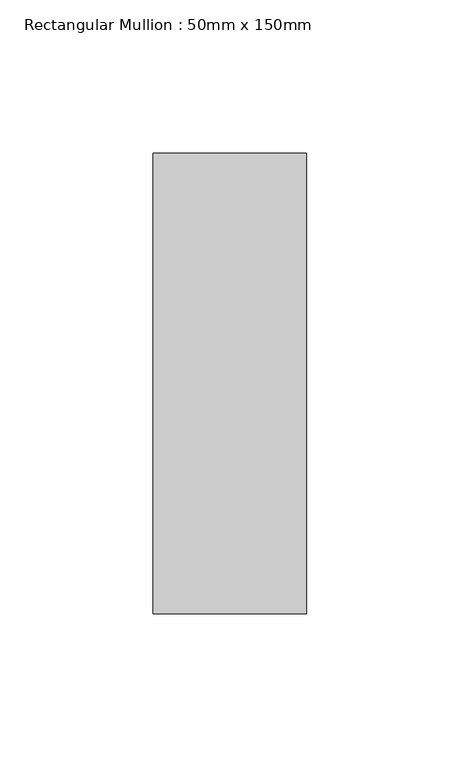
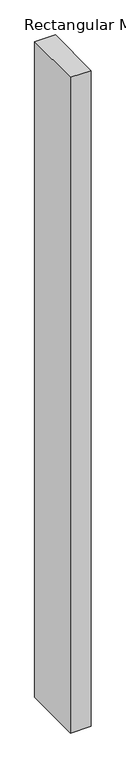
"""IFC4 building model written with IfcOpenShell, lengths in millimetres: member geometry, Rectangular Mullion : 50mm x 150mm."""

from ifc_helpers import new_model, si_unit, frame, origin, place, context, project, spatial, polyline, outline, extrude, source, transform, mapped, element, save


def rectangular_mullion_50mm_x_150mm_6fe6f3c3(model_context):
    return source(origin(), model_context, "Body", "SweptSolid", [
        extrude(outline(polyline([(0.0, 75.0), (0.0, -75.0), (-50.0, -75.0), (-50.0, 75.0), (0.0, 75.0)])), frame((0.0, 0.0, -1675.0), z_axis=(0.0, 0.0, 1.0), x_axis=(1.0, 0.0, 0.0)), (0.0, 0.0, 1.0), 1675.0),
    ])


if __name__ == "__main__":
    model = new_model("IFC4")
    model_context = context("Model", 3, world=origin())
    ifc_project = project(units=[si_unit("LENGTHUNIT", "METRE", prefix="MILLI")], contexts=[model_context])
    site = spatial("IfcSite", under=ifc_project)
    building = spatial("IfcBuilding", under=site)
    placement = place(None, origin())
    rectangular_mullion_50mm_x_150mm_shape = rectangular_mullion_50mm_x_150mm_6fe6f3c3(model_context)
    element("IfcMember", 1, ObjectType="Rectangular Mullion : 50mm x 150mm", at=placement, inside=building, context=model_context, shape_type="MappedRepresentation", body=[
        mapped(rectangular_mullion_50mm_x_150mm_shape, transform((0.0, 0.0, 0.0), x_axis=(1.0, 0.0, 0.0), y_axis=(0.0, 1.0, 0.0), z_axis=(0.0, 0.0, 1.0))),
    ])
    save(model, "model.ifc")

# Revit data of these elements
# Type "Rectangular Mullion : 50mm x 150mm"
#   built-in parameter 1007304 = 0.492126 (stored number, unit not read)
#   built-in parameter 1007301 = 0.082021 (stored number, unit not read)
#   built-in parameter 1007300 = 0.082021 (stored number, unit not read)
# Element 1 (IfcMember, "Rectangular Mullion : 50mm x 150mm")
#   Materials on its faces: "Aluminum"
# Materials
#   "Aluminum": class "Metal", colour RGB 244 244 244, transparency 0, Description = "Aluminum 6061", Cost = 0
